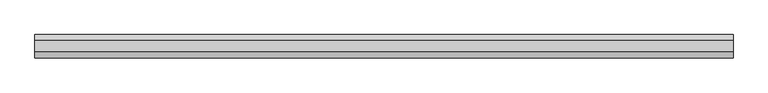
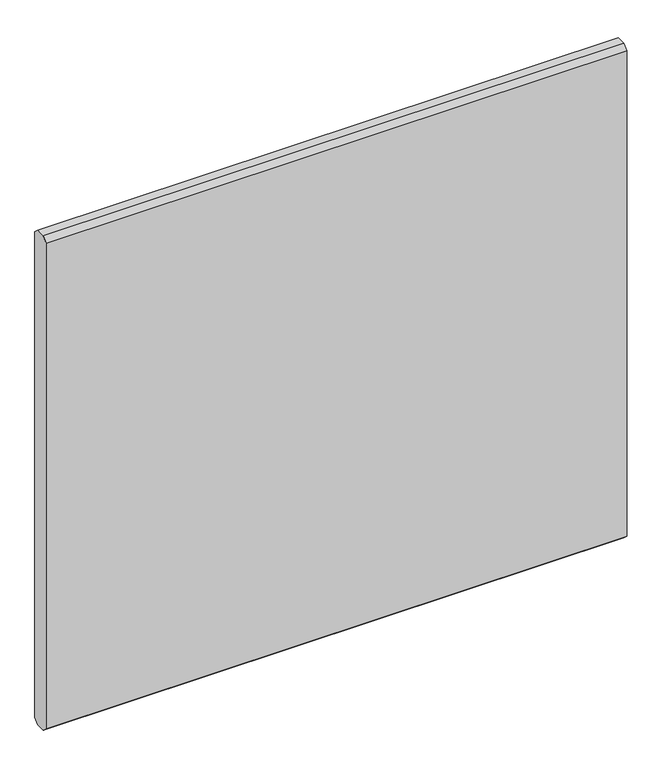
"""IFC4 building model written with IfcOpenShell, lengths in millimetres: proxy geometry, .RIPA : RIPA."""

import ifcopenshell
import ifcopenshell.guid

model = None  # the IFC model being written
_history = None  # IfcOwnerHistory: only IFC2X3 demands one
_inside = {}  # id of a spatial element -> (the spatial element, [elements in it])
_under = {}  # id of a project, library or spatial element -> (it, [spatial elements below it])
_declared = {}  # id of a project -> (the project, [libraries it declares])
_typed = {}  # id of a type object -> (the type object, [elements of that type])
_made_of = {}  # id of a material, layer set ... -> (it, [elements and type objects made of it])


def new_model(schema):
    """Start an empty IFC model of exactly this schema.

    Asked for "IFC4X3", IfcOpenShell would pick the latest addendum, in which some entities
    have other attributes; the version numbers below select the first issue.
    IFC2X3 requires an IfcOwnerHistory on every rooted entity: one is made here for all.
    """
    global model, _history
    if schema == "IFC4X3":
        model = ifcopenshell.file(schema_version=(4, 3, 0, 0))
    else:
        model = ifcopenshell.file(schema=schema)
    _inside.clear()
    _under.clear()
    _declared.clear()
    _typed.clear()
    _made_of.clear()
    _history = None
    if model.schema == "IFC2X3":
        org = make("IfcOrganization", Name="unknown")
        user = make(
            "IfcPersonAndOrganization",
            ThePerson=make("IfcPerson", FamilyName="unknown"),
            TheOrganization=org,
        )
        app = make(
            "IfcApplication",
            ApplicationDeveloper=org,
            Version="unknown",
            ApplicationFullName="unknown",
            ApplicationIdentifier="unknown",
        )
        _history = make(
            "IfcOwnerHistory",
            OwningUser=user,
            OwningApplication=app,
            ChangeAction="ADDED",
            CreationDate=0,
        )
    return model


def make(cls, **values):
    """One entity of the class cls with the attributes given. An attribute that is None is left unset."""
    return model.create_entity(
        cls, **{name: value for name, value in values.items() if value is not None}
    )


def rooted(cls, **values):
    """An entity with a GlobalId (a new one), such as an element, a storey or a relation."""
    return make(cls, GlobalId=ifcopenshell.guid.new(), OwnerHistory=_history, **values)


def si_unit(unit_type, name, prefix=None):
    """IfcSIUnit, for example si_unit("LENGTHUNIT", "METRE", prefix="MILLI")."""
    return make("IfcSIUnit", UnitType=unit_type, Prefix=prefix, Name=name)


def assignment(units):
    """IfcUnitAssignment: the units of a project."""
    return None if units is None else make("IfcUnitAssignment", Units=units)


def point(xyz):
    """IfcCartesianPoint."""
    return None if xyz is None else make("IfcCartesianPoint", Coordinates=xyz)


def direction(xyz):
    """IfcDirection."""
    return None if xyz is None else make("IfcDirection", DirectionRatios=xyz)


def frame(location, z_axis=None, x_axis=None):
    """IfcAxis2Placement3D, a coordinate frame: its origin and axes. An axis left out is left unset."""
    return make(
        "IfcAxis2Placement3D",
        Location=point(location),
        Axis=direction(z_axis),
        RefDirection=direction(x_axis),
    )


def origin():
    """The frame at (0, 0, 0) with its axes left unset."""
    return frame((0.0, 0.0, 0.0))


def place(relative_to, where):
    """IfcLocalPlacement: puts the frame where relative to a parent placement (None: the world)."""
    return make(
        "IfcLocalPlacement", PlacementRelTo=relative_to, RelativePlacement=where
    )


def context(
    kind, dimensions, precision=None, world=None, true_north=None, identifier=None
):
    """IfcGeometricRepresentationContext, for example the 3D "Model" context."""
    return make(
        "IfcGeometricRepresentationContext",
        ContextIdentifier=identifier,
        ContextType=kind,
        CoordinateSpaceDimension=dimensions,
        Precision=precision,
        WorldCoordinateSystem=world,
        TrueNorth=true_north,
    )


def project(units=None, contexts=None):
    """IfcProject with its units and contexts."""
    return rooted(
        "IfcProject",
        Name="project",
        RepresentationContexts=contexts,
        UnitsInContext=assignment(units),
    )


def spatial(cls, under=None, at=None, **own):
    """A site, building, storey or space (cls), placed at a placement, below another one or the project."""
    s = rooted(cls, ObjectPlacement=at, **own)
    if under is not None:
        _under.setdefault(under.id(), (under, []))[1].append(s)
    return s


def polyline(points):
    """IfcPolyline through the points."""
    return make("IfcPolyline", Points=[point(p) for p in points])


def outline(outer, holes=None, kind="AREA"):
    """IfcArbitraryClosedProfileDef: a profile drawn as a closed curve; with holes, ...WithVoids."""
    if holes is None:
        return make("IfcArbitraryClosedProfileDef", ProfileType=kind, OuterCurve=outer)
    return make(
        "IfcArbitraryProfileDefWithVoids",
        ProfileType=kind,
        OuterCurve=outer,
        InnerCurves=holes,
    )


def extrude(swept, where, along, depth):
    """IfcExtrudedAreaSolid: the profile swept, set in the frame where, extruded along a direction by depth."""
    return make(
        "IfcExtrudedAreaSolid",
        SweptArea=swept,
        Position=where,
        ExtrudedDirection=direction(along),
        Depth=depth,
    )


def shape(context_of_items, identifier, shape_type, items):
    """IfcShapeRepresentation: the items that make up one representation, for example the "Body"."""
    return make(
        "IfcShapeRepresentation",
        ContextOfItems=context_of_items,
        RepresentationIdentifier=identifier,
        RepresentationType=shape_type,
        Items=items,
    )


def source(mapping_origin, context_of_items, identifier, shape_type, items):
    """IfcRepresentationMap: a shape defined once, which mapped items show again and again."""
    return make(
        "IfcRepresentationMap",
        MappingOrigin=mapping_origin,
        MappedRepresentation=shape(context_of_items, identifier, shape_type, items),
    )


def transform(
    local_origin,
    x_axis=None,
    y_axis=None,
    z_axis=None,
    scale=None,
    scale2=None,
    scale3=None,
    uniform=True,
):
    """IfcCartesianTransformationOperator3D, or its non-uniform kind. x_axis, y_axis, z_axis: its Axis1, 2, 3."""
    if uniform:
        return make(
            "IfcCartesianTransformationOperator3D",
            Axis1=direction(x_axis),
            Axis2=direction(y_axis),
            LocalOrigin=point(local_origin),
            Scale=scale,
            Axis3=direction(z_axis),
        )
    return make(
        "IfcCartesianTransformationOperator3DnonUniform",
        Axis1=direction(x_axis),
        Axis2=direction(y_axis),
        LocalOrigin=point(local_origin),
        Scale=scale,
        Axis3=direction(z_axis),
        Scale2=scale2,
        Scale3=scale3,
    )


def mapped(mapping_source, mapping_target):
    """IfcMappedItem: shows the shape of a source again, moved by a transform."""
    return make(
        "IfcMappedItem", MappingSource=mapping_source, MappingTarget=mapping_target
    )


def made_of(thing, what):
    """Note that an element or type object is made of a material, layer set ...; save() writes the relation."""
    if what is not None:
        _made_of.setdefault(what.id(), (what, []))[1].append(thing)
    return thing


def element(
    cls,
    number,
    at=None,
    inside=None,
    cuts=None,
    type_object=None,
    material=None,
    context=None,
    identifier="Body",
    shape_type=None,
    held_by="IfcProductDefinitionShape",
    body=None,
    shapes=None,
    **own,
):
    """One element of the class cls, such as IfcWall. Its Tag is "e" and its number.

    at: its placement. inside: the storey or other place that contains it. cuts: it is an
    opening in that element (IfcRelVoidsElement). A single representation is given by context,
    identifier, shape_type and body (its items); several are given by shapes. held_by: the class
    of the entity that holds the representations. save() writes the other relations.
    """
    e = rooted(cls, Tag="e%d" % number, ObjectPlacement=at, **own)
    if body is not None:
        shapes = [shape(context, identifier, shape_type, body)]
    if shapes is not None:
        e.Representation = make(held_by, Representations=shapes)
    if inside is not None:
        _inside.setdefault(inside.id(), (inside, []))[1].append(e)
    if cuts is not None:
        rooted(
            "IfcRelVoidsElement", RelatingBuildingElement=cuts, RelatedOpeningElement=e
        )
    if type_object is not None:
        _typed.setdefault(type_object.id(), (type_object, []))[1].append(e)
    return made_of(e, material)


def aggregate(whole, parts):
    """IfcRelAggregates: a whole, such as a stair, and the parts it consists of."""
    return rooted("IfcRelAggregates", RelatingObject=whole, RelatedObjects=parts)


def save(model, path):
    """Write the relations noted so far, then the file.

    IfcRelAggregates (storeys below a building ...), IfcRelContainedInSpatialStructure (elements
    in a storey), IfcRelDefinesByType, IfcRelAssociatesMaterial and IfcRelDeclares: one each for
    every whole, place, type object, material and project.
    """
    for whole, parts in _under.values():
        aggregate(whole, parts)
    for where, things in _inside.values():
        rooted(
            "IfcRelContainedInSpatialStructure",
            RelatedElements=things,
            RelatingStructure=where,
        )
    for kind, things in _typed.values():
        rooted("IfcRelDefinesByType", RelatedObjects=things, RelatingType=kind)
    for what, things in _made_of.values():
        rooted("IfcRelAssociatesMaterial", RelatedObjects=things, RelatingMaterial=what)
    for by, libraries in _declared.values():
        rooted("IfcRelDeclares", RelatingContext=by, RelatedDefinitions=libraries)
    model.write(path)


def generic_models_0c544f32(model_context):
    return source(origin(), model_context, "Body", "SweptSolid", [
        extrude(outline(polyline([(-12.5, 1350.0), (12.5, 1350.0), (25.0, 1337.5), (25.0, 12.5), (12.5, 0.0), (-12.5, 0.0), (-25.0, 12.5), (-25.0, 1337.5), (-12.5, 1350.0)])), frame((-750.0, 0.0, 0.0), z_axis=(1.0, 0.0, 0.0), x_axis=(0.0, 1.0, 0.0)), (0.0, 0.0, 1.0), 1500.0),
    ])


if __name__ == "__main__":
    model = new_model("IFC4")
    model_context = context("Model", 3, world=origin())
    ifc_project = project(units=[si_unit("LENGTHUNIT", "METRE", prefix="MILLI")], contexts=[model_context])
    site = spatial("IfcSite", under=ifc_project)
    building = spatial("IfcBuilding", under=site)
    placement = place(None, origin())
    generic_models_shape = generic_models_0c544f32(model_context)
    element("IfcBuildingElementProxy", 1, Name=".RIPA : RIPA", ObjectType=".RIPA : RIPA", at=placement, inside=building, context=model_context, shape_type="MappedRepresentation", body=[
        mapped(generic_models_shape, transform((0.0, 0.0, 0.0), x_axis=(1.0, 0.0, 0.0), y_axis=(0.0, 1.0, 0.0), z_axis=(0.0, 0.0, 1.0))),
    ])
    save(model, "model.ifc")

# Revit data of these elements
# Type ".RIPA : RIPA"
#   Ripa_largura [instance default] = 0.30 m
#   Ripa_espessura [instance default] = 0.025 m
#   Ripa_comprimento [instance default] = 0.80 m
#   Ripa_chanfo [instance default] = 0.00625 m
#   Ripa_material [instance default] = none
# Element 1 (IfcBuildingElementProxy, ".RIPA : RIPA")
#   Ripa_largura = 1.35 m
#   Ripa_espessura = 0.05 m
#   Ripa_comprimento = 1.50 m
#   Ripa_chanfo = 0.0125 m
#   Ripa_material = .MADEIRA_CEREJEIRA CLARO
#   Materials on its faces: ".MADEIRA_CEREJEIRA CLARO"
# Materials
#   ".MADEIRA_CEREJEIRA CLARO": class ".CC_MADEIRA REVEST.", colour RGB 233 182 144, transparency 0, Cost = 0
